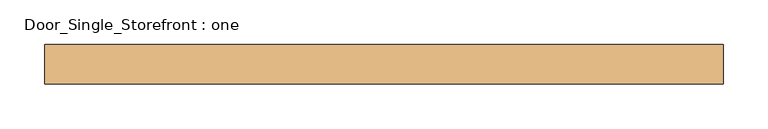
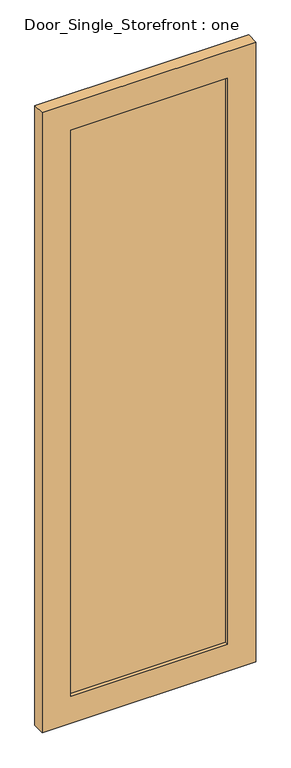
"""IFC4 building model written with IfcOpenShell, lengths in millimetres: door geometry, Door_Single_Storefront : one."""

from ifc_helpers import new_model, si_unit, frame, origin, place, context, project, spatial, polyline, outline, extrude, source, transform, mapped, element, save


def door_single_storefront_one_d7e4a69f(model_context):
    return source(origin(), model_context, "Body", "SweptSolid", [
        extrude(outline(polyline([(2336.8, -381.0), (0.0, -381.0), (0.0, 381.0), (2336.8, 381.0), (2336.8, -381.0)]), holes=[polyline([(101.6, 279.4), (101.6, -279.4), (2235.2, -279.4), (2235.2, 279.4), (101.6, 279.4)])]), frame((0.0, -50.8, 0.0), z_axis=(0.0, 1.0, 0.0), x_axis=(0.0, 0.0, 1.0)), (0.0, 0.0, 1.0), 44.45),
        extrude(outline(polyline([(279.4, -19.05), (279.4, -38.1), (-279.4, -38.1), (-279.4, -19.05), (279.4, -19.05)])), frame((0.0, 0.0, 101.6), z_axis=(0.0, 0.0, 1.0), x_axis=(1.0, 0.0, 0.0)), (0.0, 0.0, 1.0), 2133.6),
    ])


if __name__ == "__main__":
    model = new_model("IFC4")
    model_context = context("Model", 3, world=origin())
    ifc_project = project(units=[si_unit("LENGTHUNIT", "METRE", prefix="MILLI")], contexts=[model_context])
    site = spatial("IfcSite", under=ifc_project)
    building = spatial("IfcBuilding", under=site)
    placement = place(None, origin())
    door_single_storefront_one_shape = door_single_storefront_one_d7e4a69f(model_context)
    element("IfcDoor", 1, ObjectType="Door_Single_Storefront : one", at=placement, inside=building, context=model_context, shape_type="MappedRepresentation", body=[
        mapped(door_single_storefront_one_shape, transform((0.0, 0.0, 0.0), x_axis=(1.0, 0.0, 0.0), y_axis=(0.0, 1.0, 0.0), z_axis=(0.0, 0.0, 1.0))),
    ])
    save(model, "model.ifc")

# Revit data of these elements
# Type "Door_Single_Storefront : one"
#   Type Mark = "27"
#   Analytic Construction = "<None>"
#   Stile_Width = 0' - 4"
#   Door_Thickness = 0' - 1 3/4"
#   Door_Offset = 0' - 2"
#   Glass_Material = Glass
#   Frame_Material = Aluminum
#   Function = (empty or 0)
# Element 1 (IfcDoor, "Door_Single_Storefront : one")
#   Materials on its faces: "Aluminum", "Glass"
# Materials
#   "Glass": class "Glass", colour RGB 0 128 192, transparency 0.75, Description = "Soda Lime Glass", Cost = 0
#   "Aluminum": class "Metal", colour RGB 247 247 247, transparency 0, Description = "Aluminum 6061", Cost = 0
